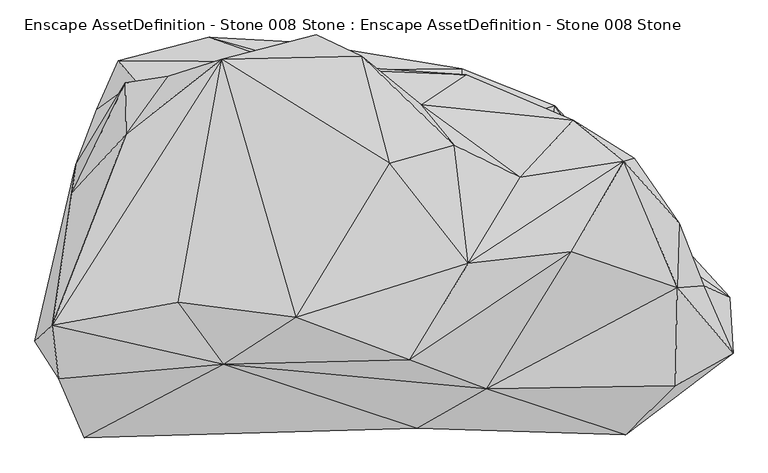
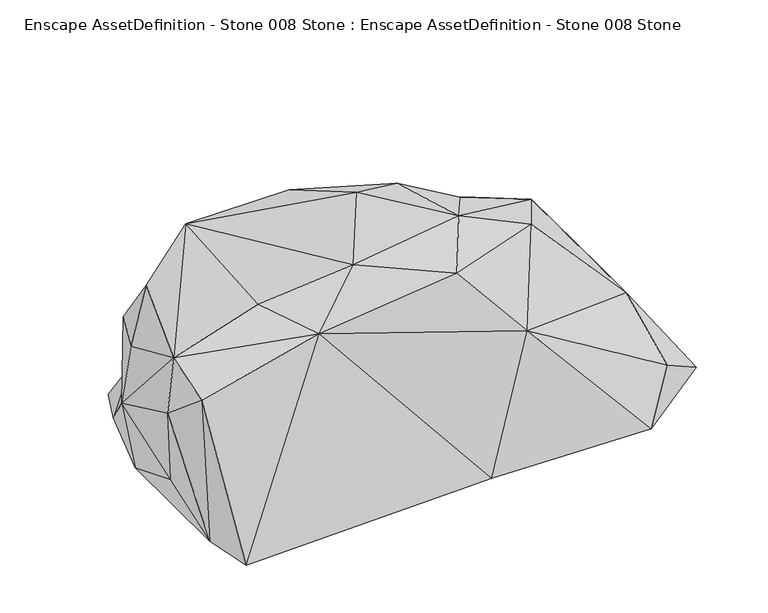
"""IFC4 building model written with IfcOpenShell, lengths in millimetres: geographic element geometry, Enscape AssetDefinition - Stone 008 Stone : Enscape AssetDefinition - Stone 008 Stone."""

from ifc_helpers import new_model, si_unit, origin, place, context, project, spatial, faceted_brep, source, transform, mapped, element, save


def enscape_assetdefinition_stone_008_stone_enscape_24533d0f(model_context):
    return source(origin(), model_context, "Body", "Brep", [
        faceted_brep([(674.4772792, 188.1209314, 142.7758336), (1035.7327461, 8.9201359, 108.4343269), (705.4293752, 497.0492125, 9.8005356), (997.1603155, 302.5434315, 403.4194052), (1162.8789902, 63.3667782, 307.4120581), (1253.1027794, -166.4617509, 132.1936697), (1349.0210772, -208.1131637, 6.9734799), (358.8430882, 390.0140226, 146.3160366), (377.8702021, 610.8905673, 436.6148412), (958.5034251, 293.037504, 588.9674425), (772.0807195, 443.9393878, 571.6524124), (1155.1955938, -174.3785888, 316.583544), (1361.7579937, -414.6891236, 4.4628736), (966.4069414, -714.6763802, 5.4843184), (1148.0065584, -535.101831, 161.3812745), (454.9190998, -545.4375148, 589.6245837), (765.6313181, -41.1196649, 728.256464), (197.4091679, -690.6881928, 2.2398918), (-514.082849, -456.0222328, 858.2776785), (170.5874205, -438.8919473, 922.1434593), (385.2636814, -83.5196525, 931.4427376), (-247.4171519, -282.6159894, 1018.4793472), (576.8572688, 233.5522175, 768.9470053), (335.1638615, 351.0840833, 853.2254696), (97.4461734, 284.5808566, 931.3715696), (213.0276859, 499.7121692, 607.2036028), (-6.4782458, 678.3997416, 740.2927279), (-523.0283737, 667.5286889, 753.1849146), (-682.7530861, -228.3637375, 932.9548478), (-874.7516274, 392.5074339, 724.0793109), (-1147.2679377, -313.0920827, 869.5514202), (-173.4227836, 757.5678229, 583.3979845), (-719.4939852, 606.0778499, 573.5012889), (-121.4118823, 631.9727302, 438.7468398), (-477.7078629, 640.0285363, 443.1231916), (-877.9751062, 580.4912448, 445.3162253), (-1074.303627, 173.3499914, 609.6158624), (-1061.0442162, 279.8386514, 242.5745577), (-839.9647474, 586.9014859, 173.4158546), (-312.4943078, 658.5144997, 220.8529711), (-903.9554596, 662.9179716, 4.3747872), (-983.217001, 483.1243753, 17.7407339), (-570.9864497, 749.253273, 0.3116064), (-136.2574697, 627.3009181, 146.1777389), (-233.8543534, 731.0650349, 7.1665621), (362.7277911, 632.3495507, 5.9714052), (-1086.7136717, 120.3676835, 13.3715561), (-1058.6297512, -132.5317025, 94.683297), (-1091.7432308, -525.1657367, 26.3983011), (-1029.1792154, -726.3221741, 1.9205989), (-1210.739255, -371.0243106, 639.5069957), (-1122.2990751, -508.4093809, 759.0334415)], [[[0, 1, 2]], [[3, 4, 1]], [[4, 5, 1]], [[1, 5, 6]], [[3, 1, 0]], [[2, 1, 6]], [[0, 2, 7]], [[7, 8, 0]], [[0, 8, 3]], [[3, 9, 4]], [[10, 3, 8]], [[3, 10, 9]], [[9, 11, 4]], [[4, 11, 5]], [[12, 5, 11]], [[12, 6, 5]], [[13, 2, 6]], [[13, 6, 12]], [[12, 11, 14]], [[12, 14, 13]], [[11, 15, 14]], [[16, 15, 11]], [[11, 9, 16]], [[14, 15, 13]], [[13, 15, 17]], [[13, 17, 2]], [[18, 15, 19]], [[16, 19, 15]], [[18, 17, 15]], [[16, 20, 19]], [[16, 9, 20]], [[21, 19, 20]], [[21, 18, 19]], [[9, 22, 20]], [[20, 22, 23]], [[20, 23, 24]], [[24, 21, 20]], [[10, 22, 9]], [[23, 22, 25]], [[25, 22, 10]], [[23, 26, 24]], [[25, 26, 23]], [[27, 21, 24]], [[27, 24, 26]], [[27, 28, 21]], [[18, 21, 28]], [[27, 29, 30]], [[27, 26, 31]], [[31, 32, 27]], [[27, 30, 28]], [[27, 32, 29]], [[26, 25, 31]], [[31, 25, 33]], [[34, 32, 31]], [[33, 34, 31]], [[32, 34, 35]], [[32, 35, 29]], [[29, 36, 30]], [[29, 35, 36]], [[35, 37, 36]], [[38, 37, 35]], [[38, 35, 34]], [[38, 34, 33]], [[25, 8, 33]], [[39, 38, 33]], [[8, 39, 33]], [[38, 40, 41]], [[37, 38, 41]], [[39, 40, 38]], [[39, 42, 40]], [[8, 43, 39]], [[42, 39, 43]], [[10, 8, 25]], [[43, 8, 7]], [[44, 43, 45]], [[44, 42, 43]], [[45, 43, 7]], [[42, 46, 41]], [[42, 41, 40]], [[46, 42, 44]], [[41, 46, 37]], [[47, 46, 48]], [[47, 37, 46]], [[46, 44, 17]], [[17, 48, 46]], [[17, 44, 45]], [[7, 2, 45]], [[17, 45, 2]], [[48, 17, 49]], [[18, 49, 17]], [[50, 48, 51]], [[47, 48, 50]], [[51, 48, 49]], [[37, 47, 50]], [[50, 51, 30]], [[50, 30, 37]], [[36, 37, 30]], [[18, 28, 30]], [[51, 18, 30]], [[49, 18, 51]]]),
    ])


if __name__ == "__main__":
    model = new_model("IFC4")
    model_context = context("Model", 3, world=origin())
    ifc_project = project(units=[si_unit("LENGTHUNIT", "METRE", prefix="MILLI")], contexts=[model_context])
    site = spatial("IfcSite", under=ifc_project)
    building = spatial("IfcBuilding", under=site)
    placement = place(None, origin())
    enscape_assetdefinition_stone_008_stone_enscape_shape = enscape_assetdefinition_stone_008_stone_enscape_24533d0f(model_context)
    element("IfcGeographicElement", 1, ObjectType="Enscape AssetDefinition - Stone 008 Stone : Enscape AssetDefinition - Stone 008 Stone", at=placement, inside=building, context=model_context, shape_type="MappedRepresentation", body=[
        mapped(enscape_assetdefinition_stone_008_stone_enscape_shape, transform((0.0, 0.0, 0.0), x_axis=(1.0, 0.0, 0.0), y_axis=(0.0, 1.0, 0.0), z_axis=(0.0, 0.0, 1.0))),
    ])
    save(model, "model.ifc")

# Revit data of these elements
# Type "Enscape AssetDefinition - Stone 008 Stone : Enscape AssetDefinition - Stone 008 Stone"
#   EnscapeAssetSource = "REMOTE"
#   EnscapeAssetId = "21c0a78a-166e-4c5c-8e35-d18d7a930555"
#   Height = 1.018479 m
#   EnscapeNativeAssetHeight = 1.018479 m
#   Default Elevation = 0
